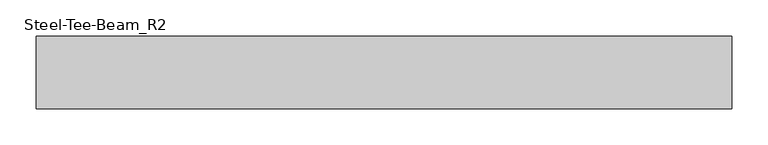
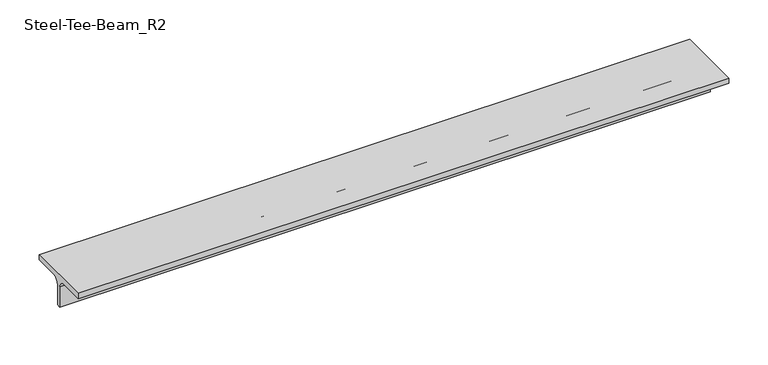
"""IFC4 building model written with IfcOpenShell, lengths in millimetres: beam geometry, Steel-Tee-Beam_R2 : BM127_CT-50x100x6x8_TB1."""

import ifcopenshell
import ifcopenshell.guid

model = None  # the IFC model being written
_history = None  # IfcOwnerHistory: only IFC2X3 demands one
_inside = {}  # id of a spatial element -> (the spatial element, [elements in it])
_under = {}  # id of a project, library or spatial element -> (it, [spatial elements below it])
_declared = {}  # id of a project -> (the project, [libraries it declares])
_typed = {}  # id of a type object -> (the type object, [elements of that type])
_made_of = {}  # id of a material, layer set ... -> (it, [elements and type objects made of it])


def new_model(schema):
    """Start an empty IFC model of exactly this schema.

    Asked for "IFC4X3", IfcOpenShell would pick the latest addendum, in which some entities
    have other attributes; the version numbers below select the first issue.
    IFC2X3 requires an IfcOwnerHistory on every rooted entity: one is made here for all.
    """
    global model, _history
    if schema == "IFC4X3":
        model = ifcopenshell.file(schema_version=(4, 3, 0, 0))
    else:
        model = ifcopenshell.file(schema=schema)
    _inside.clear()
    _under.clear()
    _declared.clear()
    _typed.clear()
    _made_of.clear()
    _history = None
    if model.schema == "IFC2X3":
        org = make("IfcOrganization", Name="unknown")
        user = make(
            "IfcPersonAndOrganization",
            ThePerson=make("IfcPerson", FamilyName="unknown"),
            TheOrganization=org,
        )
        app = make(
            "IfcApplication",
            ApplicationDeveloper=org,
            Version="unknown",
            ApplicationFullName="unknown",
            ApplicationIdentifier="unknown",
        )
        _history = make(
            "IfcOwnerHistory",
            OwningUser=user,
            OwningApplication=app,
            ChangeAction="ADDED",
            CreationDate=0,
        )
    return model


def make(cls, **values):
    """One entity of the class cls with the attributes given. An attribute that is None is left unset."""
    return model.create_entity(
        cls, **{name: value for name, value in values.items() if value is not None}
    )


def rooted(cls, **values):
    """An entity with a GlobalId (a new one), such as an element, a storey or a relation."""
    return make(cls, GlobalId=ifcopenshell.guid.new(), OwnerHistory=_history, **values)


def si_unit(unit_type, name, prefix=None):
    """IfcSIUnit, for example si_unit("LENGTHUNIT", "METRE", prefix="MILLI")."""
    return make("IfcSIUnit", UnitType=unit_type, Prefix=prefix, Name=name)


def assignment(units):
    """IfcUnitAssignment: the units of a project."""
    return None if units is None else make("IfcUnitAssignment", Units=units)


def point(xyz):
    """IfcCartesianPoint."""
    return None if xyz is None else make("IfcCartesianPoint", Coordinates=xyz)


def direction(xyz):
    """IfcDirection."""
    return None if xyz is None else make("IfcDirection", DirectionRatios=xyz)


def frame(location, z_axis=None, x_axis=None):
    """IfcAxis2Placement3D, a coordinate frame: its origin and axes. An axis left out is left unset."""
    return make(
        "IfcAxis2Placement3D",
        Location=point(location),
        Axis=direction(z_axis),
        RefDirection=direction(x_axis),
    )


def frame_2d(location, x_axis=None):
    """IfcAxis2Placement2D, a coordinate frame in the plane: its origin and x axis."""
    return make(
        "IfcAxis2Placement2D", Location=point(location), RefDirection=direction(x_axis)
    )


def origin():
    """The frame at (0, 0, 0) with its axes left unset."""
    return frame((0.0, 0.0, 0.0))


def place(relative_to, where):
    """IfcLocalPlacement: puts the frame where relative to a parent placement (None: the world)."""
    return make(
        "IfcLocalPlacement", PlacementRelTo=relative_to, RelativePlacement=where
    )


def context(
    kind, dimensions, precision=None, world=None, true_north=None, identifier=None
):
    """IfcGeometricRepresentationContext, for example the 3D "Model" context."""
    return make(
        "IfcGeometricRepresentationContext",
        ContextIdentifier=identifier,
        ContextType=kind,
        CoordinateSpaceDimension=dimensions,
        Precision=precision,
        WorldCoordinateSystem=world,
        TrueNorth=true_north,
    )


def project(units=None, contexts=None):
    """IfcProject with its units and contexts."""
    return rooted(
        "IfcProject",
        Name="project",
        RepresentationContexts=contexts,
        UnitsInContext=assignment(units),
    )


def spatial(cls, under=None, at=None, **own):
    """A site, building, storey or space (cls), placed at a placement, below another one or the project."""
    s = rooted(cls, ObjectPlacement=at, **own)
    if under is not None:
        _under.setdefault(under.id(), (under, []))[1].append(s)
    return s


def polyline(points):
    """IfcPolyline through the points."""
    return make("IfcPolyline", Points=[point(p) for p in points])


def circle_curve(where, radius):
    """IfcCircle in the frame where."""
    return make("IfcCircle", Position=where, Radius=radius)


def trimmed(basis, trim1, trim2, sense, master):
    """IfcTrimmedCurve: the piece of a basis curve between two trims."""
    return make(
        "IfcTrimmedCurve",
        BasisCurve=basis,
        Trim1=trim1,
        Trim2=trim2,
        SenseAgreement=sense,
        MasterRepresentation=master,
    )


def segment(curve, same_sense, transition):
    """IfcCompositeCurveSegment."""
    return make(
        "IfcCompositeCurveSegment",
        Transition=transition,
        SameSense=same_sense,
        ParentCurve=curve,
    )


def composite_curve(segments, self_intersect=None):
    """IfcCompositeCurve: segments joined end to end."""
    return make("IfcCompositeCurve", Segments=segments, SelfIntersect=self_intersect)


def outline(outer, holes=None, kind="AREA"):
    """IfcArbitraryClosedProfileDef: a profile drawn as a closed curve; with holes, ...WithVoids."""
    if holes is None:
        return make("IfcArbitraryClosedProfileDef", ProfileType=kind, OuterCurve=outer)
    return make(
        "IfcArbitraryProfileDefWithVoids",
        ProfileType=kind,
        OuterCurve=outer,
        InnerCurves=holes,
    )


def extrude(swept, where, along, depth):
    """IfcExtrudedAreaSolid: the profile swept, set in the frame where, extruded along a direction by depth."""
    return make(
        "IfcExtrudedAreaSolid",
        SweptArea=swept,
        Position=where,
        ExtrudedDirection=direction(along),
        Depth=depth,
    )


def shape(context_of_items, identifier, shape_type, items):
    """IfcShapeRepresentation: the items that make up one representation, for example the "Body"."""
    return make(
        "IfcShapeRepresentation",
        ContextOfItems=context_of_items,
        RepresentationIdentifier=identifier,
        RepresentationType=shape_type,
        Items=items,
    )


def source(mapping_origin, context_of_items, identifier, shape_type, items):
    """IfcRepresentationMap: a shape defined once, which mapped items show again and again."""
    return make(
        "IfcRepresentationMap",
        MappingOrigin=mapping_origin,
        MappedRepresentation=shape(context_of_items, identifier, shape_type, items),
    )


def transform(
    local_origin,
    x_axis=None,
    y_axis=None,
    z_axis=None,
    scale=None,
    scale2=None,
    scale3=None,
    uniform=True,
):
    """IfcCartesianTransformationOperator3D, or its non-uniform kind. x_axis, y_axis, z_axis: its Axis1, 2, 3."""
    if uniform:
        return make(
            "IfcCartesianTransformationOperator3D",
            Axis1=direction(x_axis),
            Axis2=direction(y_axis),
            LocalOrigin=point(local_origin),
            Scale=scale,
            Axis3=direction(z_axis),
        )
    return make(
        "IfcCartesianTransformationOperator3DnonUniform",
        Axis1=direction(x_axis),
        Axis2=direction(y_axis),
        LocalOrigin=point(local_origin),
        Scale=scale,
        Axis3=direction(z_axis),
        Scale2=scale2,
        Scale3=scale3,
    )


def mapped(mapping_source, mapping_target):
    """IfcMappedItem: shows the shape of a source again, moved by a transform."""
    return make(
        "IfcMappedItem", MappingSource=mapping_source, MappingTarget=mapping_target
    )


def made_of(thing, what):
    """Note that an element or type object is made of a material, layer set ...; save() writes the relation."""
    if what is not None:
        _made_of.setdefault(what.id(), (what, []))[1].append(thing)
    return thing


def element(
    cls,
    number,
    at=None,
    inside=None,
    cuts=None,
    type_object=None,
    material=None,
    context=None,
    identifier="Body",
    shape_type=None,
    held_by="IfcProductDefinitionShape",
    body=None,
    shapes=None,
    **own,
):
    """One element of the class cls, such as IfcWall. Its Tag is "e" and its number.

    at: its placement. inside: the storey or other place that contains it. cuts: it is an
    opening in that element (IfcRelVoidsElement). A single representation is given by context,
    identifier, shape_type and body (its items); several are given by shapes. held_by: the class
    of the entity that holds the representations. save() writes the other relations.
    """
    e = rooted(cls, Tag="e%d" % number, ObjectPlacement=at, **own)
    if body is not None:
        shapes = [shape(context, identifier, shape_type, body)]
    if shapes is not None:
        e.Representation = make(held_by, Representations=shapes)
    if inside is not None:
        _inside.setdefault(inside.id(), (inside, []))[1].append(e)
    if cuts is not None:
        rooted(
            "IfcRelVoidsElement", RelatingBuildingElement=cuts, RelatedOpeningElement=e
        )
    if type_object is not None:
        _typed.setdefault(type_object.id(), (type_object, []))[1].append(e)
    return made_of(e, material)


def aggregate(whole, parts):
    """IfcRelAggregates: a whole, such as a stair, and the parts it consists of."""
    return rooted("IfcRelAggregates", RelatingObject=whole, RelatedObjects=parts)


def save(model, path):
    """Write the relations noted so far, then the file.

    IfcRelAggregates (storeys below a building ...), IfcRelContainedInSpatialStructure (elements
    in a storey), IfcRelDefinesByType, IfcRelAssociatesMaterial and IfcRelDeclares: one each for
    every whole, place, type object, material and project.
    """
    for whole, parts in _under.values():
        aggregate(whole, parts)
    for where, things in _inside.values():
        rooted(
            "IfcRelContainedInSpatialStructure",
            RelatedElements=things,
            RelatingStructure=where,
        )
    for kind, things in _typed.values():
        rooted("IfcRelDefinesByType", RelatedObjects=things, RelatingType=kind)
    for what, things in _made_of.values():
        rooted("IfcRelAssociatesMaterial", RelatedObjects=things, RelatingMaterial=what)
    for by, libraries in _declared.values():
        rooted("IfcRelDeclares", RelatingContext=by, RelatedDefinitions=libraries)
    model.write(path)


def steel_tee_beam_r2_b2c95b6f(model_context):
    return source(origin(), model_context, "Body", "SweptSolid", [
        extrude(outline(composite_curve([segment(polyline([(-50.0, 25.0), (50.0, 25.0), (50.0, 17.0), (13.0, 17.0)]), True, "CONTINUOUS"), segment(trimmed(circle_curve(frame_2d((13.0, 7.0)), 10.0), [point((13.0, 17.0))], [point((3.0, 7.0))], True, "CARTESIAN"), True, "CONTINUOUS"), segment(polyline([(3.0, 7.0), (3.0, -25.0), (-3.0, -25.0), (-3.0, 7.0)]), True, "CONTINUOUS"), segment(trimmed(circle_curve(frame_2d((-13.0, 7.0)), 10.0), [point((-3.0, 7.0))], [point((-13.0, 17.0))], True, "CARTESIAN"), True, "CONTINUOUS"), segment(polyline([(-13.0, 17.0), (-50.0, 17.0), (-50.0, 25.0)]), True, "CONTINUOUS")], self_intersect=False)), frame((-480.0, 0.0, 0.0), z_axis=(1.0, 0.0, 0.0), x_axis=(0.0, 1.0, 0.0)), (0.0, 0.0, 1.0), 960.0),
    ])


if __name__ == "__main__":
    model = new_model("IFC4")
    model_context = context("Model", 3, world=origin())
    ifc_project = project(units=[si_unit("LENGTHUNIT", "METRE", prefix="MILLI")], contexts=[model_context])
    site = spatial("IfcSite", under=ifc_project)
    building = spatial("IfcBuilding", under=site)
    placement = place(None, origin())
    steel_tee_beam_r2_shape = steel_tee_beam_r2_b2c95b6f(model_context)
    element("IfcBeam", 1, ObjectType="Steel-Tee-Beam_R2 : BM127_CT-50x100x6x8_TB1", at=placement, inside=building, context=model_context, shape_type="MappedRepresentation", body=[
        mapped(steel_tee_beam_r2_shape, transform((0.0, 0.0, 0.0), x_axis=(1.0, 0.0, 0.0), y_axis=(0.0, 1.0, 0.0), z_axis=(0.0, 0.0, 1.0))),
    ])
    save(model, "model.ifc")

# Revit data of these elements
# Type "Steel-Tee-Beam_R2 : BM127_CT-50x100x6x8_TB1"
#   SteelWeight = "Light"
#   Surface Area = 0.291416 m²/m
#   Section Area = 10.9492 cm²
#   Mass per Unit Length = 8.59512 kg/m
#   Length [instance default] = 1524 mm
#   bf = 100 mm
#   d = 50 mm
#   k = 18 mm
#   r = 10 mm
#   tf = 8 mm
#   tw = 6 mm
#   hec_material4 [instance default] = none
#   hec_material3 [instance default] = none
#   hec_material2 [instance default] = none
#   hec_material1 [instance default] = none
#   Structural Material [instance default] = Steel, 45-345
#   Assembly Code = ""
# Element 1 (IfcBeam, "Steel-Tee-Beam_R2 : BM127_CT-50x100x6x8_TB1")
#   Materials on its faces: "Steel, 45-345"
# Materials
#   "Steel, 45-345": class "Metal", colour RGB 189 187 185, transparency 0, Description = "Steel 345 MPa", Cost = 0
